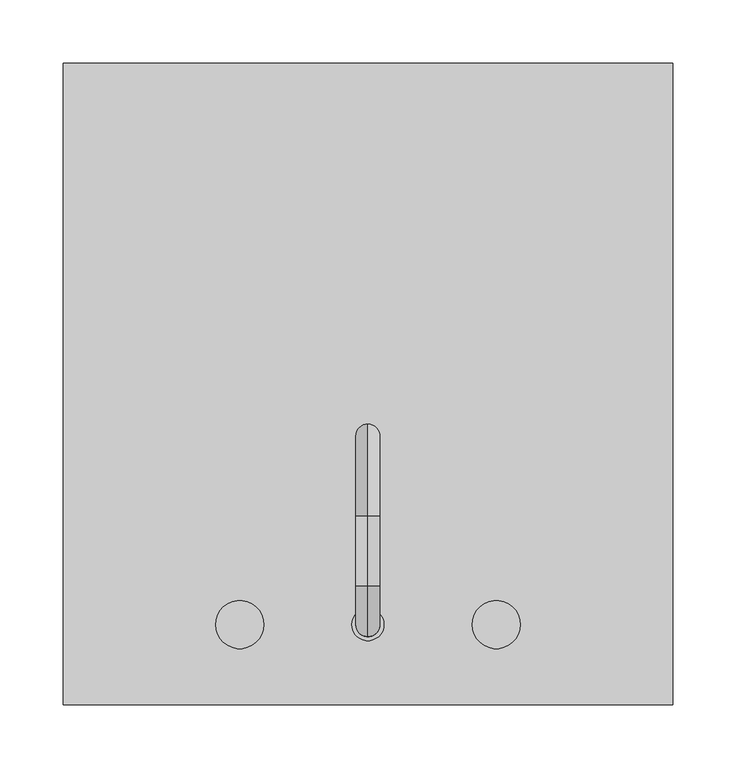
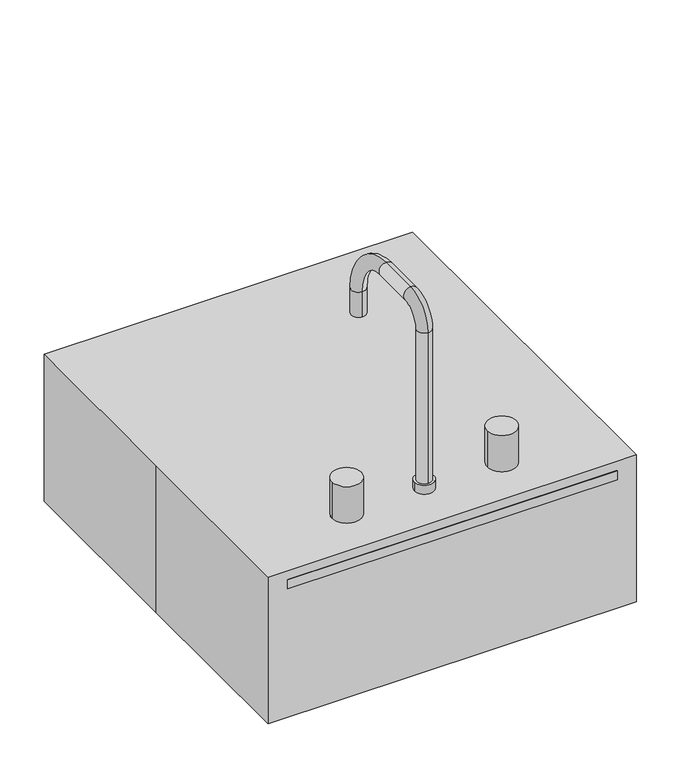
"""IFC4 building model written with IfcOpenShell, lengths in millimetres: proxy geometry, CS040 - Sink, SS, Single Compartment, 7.5x14x14 ID : CS040 - Sink, SS, Single Compartment, 7.5x14x14 ID."""

from ifc_helpers import new_model, si_unit, point, frame, frame_2d, origin, origin_with_axes, place, context, project, spatial, polyline, circle_curve, ellipse_curve, trimmed, segment, composite_curve, outline, extrude, source, transform, mapped, element, save
from ifc_brep_helpers import plane_surface, cylinder_surface, revolved_surface, advanced_brep


def specialty_equipment_c9b423af(model_context):
    return source(origin(), model_context, "Body", "SolidModel", [
        advanced_brep(
        [(-215.9, 215.9, 190.5), (-215.9, -254.0, 190.5), (215.9, -254.0, 190.5), (215.9, 215.9, 190.5), (133.35, -139.7, 190.5), (-133.35, -139.7, 190.5), (-177.8, -95.25, 190.5), (-177.8, 133.35, 190.5), (-133.35, 177.8, 190.5), (133.35, 177.8, 190.5), (177.8, 133.35, 190.5), (177.8, -95.25, 190.5), (-120.65, -190.5, 190.5), (-82.55, -190.5, 190.5), (-19.05, -190.5, 190.5), (19.05, -190.5, 190.5), (82.55, -190.5, 190.5), (120.65, -190.5, 190.5), (-215.9, 215.9, 177.8), (215.9, 215.9, 177.8), (215.9, -254.0, 177.8), (-215.9, -254.0, 177.8), (-120.65, -190.5, 177.8), (-82.55, -190.5, 177.8), (-19.05, -190.5, 177.8), (19.05, -190.5, 177.8), (82.55, -190.5, 177.8), (120.65, -190.5, 177.8), (184.15, -95.25, 177.8), (184.15, 133.35, 177.8), (133.35, 184.15, 177.8), (-133.35, 184.15, 177.8), (-184.15, 133.35, 177.8), (-184.15, -95.25, 177.8), (-133.35, -146.05, 177.8), (133.35, -146.05, 177.8), (177.8, -95.25, 177.8), (133.35, -139.7, 177.8), (177.8, 133.35, 177.8), (177.8, 133.35, 6.35), (177.8, -95.25, 6.35), (133.35, 177.8, 177.8), (-133.35, 177.8, 177.8), (-133.35, 177.8, 6.35), (133.35, 177.8, 6.35), (-177.8, 133.35, 177.8), (-177.8, -95.25, 177.8), (-177.8, -95.25, 6.35), (-177.8, 133.35, 6.35), (-133.35, -139.7, 177.8), (133.35, -139.7, 6.35), (-133.35, -139.7, 6.35), (184.15, -95.25, 0.0), (133.35, -146.05, 0.0), (184.15, 133.35, 0.0), (133.35, 184.15, 0.0), (-133.35, 184.15, 0.0), (-184.15, 133.35, 0.0), (-184.15, -95.25, 0.0), (-133.35, -146.05, 0.0), (-19.05, 19.05, 0.0), (19.05, 19.05, 0.0), (-19.05, 19.05, 6.35), (19.05, 19.05, 6.35)],
        [
            (0, 1),
            (1, 2),
            (2, 3),
            (3, 0),
            (4, 5),
            (5, 6, circle_curve(frame((-133.35, -95.25, 190.5), z_axis=(0.0, 0.0, -1.0), x_axis=(1.0, 0.0, 0.0)), 44.45)),
            (6, 7),
            (7, 8, circle_curve(frame((-133.35, 133.35, 190.5), z_axis=(0.0, 0.0, -1.0), x_axis=(1.0, 0.0, 0.0)), 44.45)),
            (8, 9),
            (9, 10, circle_curve(frame((133.35, 133.35, 190.5), z_axis=(0.0, 0.0, -1.0), x_axis=(1.0, 0.0, 0.0)), 44.45)),
            (10, 11),
            (11, 4, circle_curve(frame((133.35, -95.25, 190.5), z_axis=(0.0, 0.0, -1.0), x_axis=(1.0, 0.0, 0.0)), 44.45)),
            (12, 13, circle_curve(frame((-101.6, -190.5, 190.5), z_axis=(0.0, 0.0, -1.0), x_axis=(1.0, 0.0, 0.0)), 19.05)),
            (13, 12, circle_curve(frame((-101.6, -190.5, 190.5), z_axis=(0.0, 0.0, -1.0), x_axis=(1.0, 0.0, 0.0)), 19.05)),
            (14, 15, circle_curve(frame((0.0, -190.5, 190.5), z_axis=(0.0, 0.0, -1.0), x_axis=(1.0, 0.0, 0.0)), 19.05)),
            (15, 14, circle_curve(frame((0.0, -190.5, 190.5), z_axis=(0.0, 0.0, -1.0), x_axis=(1.0, 0.0, 0.0)), 19.05)),
            (16, 17, circle_curve(frame((101.6, -190.5, 190.5), z_axis=(0.0, 0.0, -1.0), x_axis=(1.0, 0.0, 0.0)), 19.05)),
            (17, 16, circle_curve(frame((101.6, -190.5, 190.5), z_axis=(0.0, 0.0, -1.0), x_axis=(1.0, 0.0, 0.0)), 19.05)),
            (18, 19),
            (19, 20),
            (20, 21),
            (21, 18),
            (22, 23, circle_curve(frame((-101.6, -190.5, 177.8), z_axis=(0.0, 0.0, 1.0), x_axis=(1.0, 0.0, 0.0)), 19.05)),
            (23, 22, circle_curve(frame((-101.6, -190.5, 177.8), z_axis=(0.0, 0.0, 1.0), x_axis=(1.0, 0.0, 0.0)), 19.05)),
            (24, 25, circle_curve(frame((0.0, -190.5, 177.8), z_axis=(0.0, 0.0, 1.0), x_axis=(1.0, 0.0, 0.0)), 19.05)),
            (25, 24, circle_curve(frame((0.0, -190.5, 177.8), z_axis=(0.0, 0.0, 1.0), x_axis=(1.0, 0.0, 0.0)), 19.05)),
            (26, 27, circle_curve(frame((101.6, -190.5, 177.8), z_axis=(0.0, 0.0, 1.0), x_axis=(1.0, 0.0, 0.0)), 19.05)),
            (27, 26, circle_curve(frame((101.6, -190.5, 177.8), z_axis=(0.0, 0.0, 1.0), x_axis=(1.0, 0.0, 0.0)), 19.05)),
            (28, 29),
            (29, 30, circle_curve(frame((133.35, 133.35, 177.8), z_axis=(0.0, 0.0, 1.0), x_axis=(1.0, 0.0, 0.0)), 50.8)),
            (30, 31),
            (31, 32, circle_curve(frame((-133.35, 133.35, 177.8), z_axis=(0.0, 0.0, 1.0), x_axis=(0.0, 1.0, 0.0)), 50.8)),
            (32, 33),
            (33, 34, circle_curve(frame((-133.35, -95.25, 177.8), z_axis=(0.0, 0.0, 1.0), x_axis=(-1.0, 0.0, 0.0)), 50.8)),
            (34, 35),
            (35, 28, circle_curve(frame((133.35, -95.25, 177.8), z_axis=(0.0, 0.0, 1.0), x_axis=(0.0, -1.0, 0.0)), 50.8)),
            (3, 19),
            (18, 0),
            (2, 20),
            (1, 21),
            (11, 36),
            (36, 37, circle_curve(frame((133.35, -95.25, 177.8), z_axis=(0.0, 0.0, -1.0), x_axis=(1.0, 0.0, 0.0)), 44.45)),
            (37, 4),
            (10, 38),
            (38, 39),
            (39, 40),
            (40, 36),
            (9, 41),
            (41, 38, circle_curve(frame((133.35, 133.35, 177.8), z_axis=(0.0, 0.0, -1.0), x_axis=(1.0, 0.0, 0.0)), 44.45)),
            (8, 42),
            (42, 43),
            (43, 44),
            (44, 41),
            (7, 45),
            (45, 42, circle_curve(frame((-133.35, 133.35, 177.8), z_axis=(0.0, 0.0, -1.0), x_axis=(1.0, 0.0, 0.0)), 44.45)),
            (6, 46),
            (46, 47),
            (47, 48),
            (48, 45),
            (5, 49),
            (49, 46, circle_curve(frame((-133.35, -95.25, 177.8), z_axis=(0.0, 0.0, -1.0), x_axis=(1.0, 0.0, 0.0)), 44.45)),
            (37, 50),
            (50, 51),
            (51, 49),
            (13, 23),
            (22, 12),
            (15, 25),
            (24, 14),
            (17, 27),
            (26, 16),
            (52, 28),
            (35, 53),
            (53, 52, circle_curve(frame((133.35, -95.25, 0.0), z_axis=(0.0, 0.0, 1.0), x_axis=(0.0, -1.0, 0.0)), 50.8)),
            (40, 50, circle_curve(frame((133.35, -95.25, 6.35), z_axis=(0.0, 0.0, -1.0), x_axis=(0.0, -1.0, 0.0)), 44.45)),
            (52, 54),
            (54, 29),
            (54, 55, circle_curve(frame((133.35, 133.35, 0.0), z_axis=(0.0, 0.0, 1.0), x_axis=(1.0, 0.0, 0.0)), 50.8)),
            (55, 30),
            (44, 39, circle_curve(frame((133.35, 133.35, 6.35), z_axis=(0.0, 0.0, -1.0), x_axis=(1.0, 0.0, 0.0)), 44.45)),
            (55, 56),
            (56, 31),
            (56, 57, circle_curve(frame((-133.35, 133.35, 0.0), z_axis=(0.0, 0.0, 1.0), x_axis=(0.0, 1.0, 0.0)), 50.8)),
            (57, 32),
            (48, 43, circle_curve(frame((-133.35, 133.35, 6.35), z_axis=(0.0, 0.0, -1.0), x_axis=(0.0, 1.0, 0.0)), 44.45)),
            (57, 58),
            (58, 33),
            (58, 59, circle_curve(frame((-133.35, -95.25, 0.0), z_axis=(0.0, 0.0, 1.0), x_axis=(-1.0, 0.0, 0.0)), 50.8)),
            (59, 34),
            (51, 47, circle_curve(frame((-133.35, -95.25, 6.35), z_axis=(0.0, 0.0, -1.0), x_axis=(-1.0, 0.0, 0.0)), 44.45)),
            (59, 53),
            (60, 61, circle_curve(frame((0.0, 19.05, 0.0), z_axis=(0.0, 0.0, 1.0), x_axis=(1.0, 0.0, 0.0)), 19.05)),
            (61, 60, circle_curve(frame((0.0, 19.05, 0.0), z_axis=(0.0, 0.0, 1.0), x_axis=(1.0, 0.0, 0.0)), 19.05)),
            (62, 63, circle_curve(frame((0.0, 19.05, 6.35), z_axis=(0.0, 0.0, -1.0), x_axis=(1.0, 0.0, 0.0)), 19.05)),
            (63, 62, circle_curve(frame((0.0, 19.05, 6.35), z_axis=(0.0, 0.0, -1.0), x_axis=(1.0, 0.0, 0.0)), 19.05)),
            (63, 61),
            (60, 62),
        ],
        [
            plane_surface(frame((215.9, 215.9, 190.5), z_axis=(0.0, 0.0, 1.0), x_axis=(1.0, 0.0, 0.0))),
            plane_surface(frame((215.9, 215.9, 177.8), z_axis=(0.0, 0.0, -1.0), x_axis=(-1.0, 0.0, 0.0))),
            plane_surface(frame((-215.9, 215.9, 190.5), z_axis=(0.0, 1.0, 0.0), x_axis=(0.0, 0.0, -1.0))),
            plane_surface(frame((215.9, 215.9, 190.5), z_axis=(1.0, 0.0, 0.0), x_axis=(0.0, 0.0, -1.0))),
            plane_surface(frame((215.9, -254.0, 190.5), z_axis=(0.0, -1.0, 0.0), x_axis=(0.0, 0.0, -1.0))),
            plane_surface(frame((-215.9, -254.0, 190.5), z_axis=(-1.0, 0.0, 0.0), x_axis=(0.0, 0.0, -1.0))),
            revolved_surface(polyline([(177.8, -95.25, 177.8), (177.8, -95.25, 190.5)]), (133.35, -95.25, 177.8), (0.0, 0.0, -1.0)),
            plane_surface(frame((177.8, -95.25, 190.5), z_axis=(-1.0, 0.0, 0.0), x_axis=(0.0, 0.0, -1.0))),
            revolved_surface(polyline([(177.8, 133.35, 177.8), (177.8, 133.35, 190.5)]), (133.35, 133.35, 177.8), (0.0, 0.0, -1.0)),
            plane_surface(frame((133.35, 177.8, 190.5), z_axis=(0.0, -1.0, 0.0), x_axis=(0.0, 0.0, -1.0))),
            revolved_surface(polyline([(-88.89999999999999, 133.35, 177.8), (-88.89999999999999, 133.35, 190.5)]), (-133.35, 133.35, 177.8), (0.0, 0.0, -1.0)),
            plane_surface(frame((-177.8, 133.35, 190.5), z_axis=(1.0, 0.0, 0.0), x_axis=(0.0, 0.0, -1.0))),
            revolved_surface(polyline([(-88.89999999999999, -95.25, 177.8), (-88.89999999999999, -95.25, 190.5)]), (-133.35, -95.25, 177.8), (0.0, 0.0, -1.0)),
            plane_surface(frame((-133.35, -139.7, 190.5), z_axis=(0.0, 1.0, 0.0), x_axis=(0.0, 0.0, -1.0))),
            revolved_surface(polyline([(-82.55, -190.5, 177.8), (-82.55, -190.5, 190.5)]), (-101.6, -190.5, 177.8), (0.0, 0.0, -1.0)),
            revolved_surface(polyline([(19.05, -190.5, 177.8), (19.05, -190.5, 190.5)]), (0.0, -190.5, 177.8), (0.0, 0.0, -1.0)),
            revolved_surface(polyline([(120.64999999999999, -190.5, 177.8), (120.64999999999999, -190.5, 190.5)]), (101.6, -190.5, 177.8), (0.0, 0.0, -1.0)),
            cylinder_surface(frame((133.35, -95.25, 190.5), z_axis=(0.0, 0.0, -1.0), x_axis=(0.0, -1.0, 0.0)), 50.8),
            revolved_surface(polyline([(133.35, -139.7, 6.349999999999994), (133.35, -139.7, 177.8)]), (133.35, -95.25, 190.5), (0.0, 0.0, -1.0)),
            plane_surface(frame((184.15, -95.25, 177.8), z_axis=(1.0, 0.0, 0.0), x_axis=(0.0, 1.0, 0.0))),
            cylinder_surface(frame((133.35, 133.35, 190.5), z_axis=(0.0, 0.0, -1.0), x_axis=(1.0, 0.0, 0.0)), 50.8),
            revolved_surface(polyline([(177.8, 133.35, 6.349999999999994), (177.8, 133.35, 177.8)]), (133.35, 133.35, 190.5), (0.0, 0.0, -1.0)),
            plane_surface(frame((133.35, 184.15, 177.8), z_axis=(0.0, 1.0, 0.0), x_axis=(-1.0, 0.0, 0.0))),
            cylinder_surface(frame((-133.35, 133.35, 190.5), z_axis=(0.0, 0.0, -1.0), x_axis=(0.0, 1.0, 0.0)), 50.8),
            revolved_surface(polyline([(-133.35, 177.8, 6.349999999999994), (-133.35, 177.8, 177.8)]), (-133.35, 133.35, 190.5), (0.0, 0.0, -1.0)),
            plane_surface(frame((-184.15, 133.35, 177.8), z_axis=(-1.0, 0.0, 0.0), x_axis=(0.0, -1.0, 0.0))),
            cylinder_surface(frame((-133.35, -95.25, 190.5), z_axis=(0.0, 0.0, -1.0), x_axis=(-1.0, 0.0, 0.0)), 50.8),
            revolved_surface(polyline([(-177.8, -95.25, 6.349999999999994), (-177.8, -95.25, 177.8)]), (-133.35, -95.25, 190.5), (0.0, 0.0, -1.0)),
            plane_surface(frame((-133.35, -146.05, 177.8), z_axis=(0.0, -1.0, 0.0), x_axis=(1.0, 0.0, 0.0))),
            plane_surface(frame((-133.35, -146.05, 0.0), z_axis=(0.0, 0.0, -1.0), x_axis=(1.0, 0.0, 0.0))),
            plane_surface(frame((-88.9, -95.25, 6.35), z_axis=(0.0, 0.0, 1.0), x_axis=(0.0, -1.0, 0.0))),
            revolved_surface(polyline([(19.05, 19.05, 0.0), (19.05, 19.05, 6.35)]), (0.0, 19.05, 0.0), (0.0, 0.0, -1.0)),
        ],
        [
            (0, [[1, 2, 3, 4], [5, 6, 7, 8, 9, 10, 11, 12], [13, 14], [15, 16], [17, 18]]),
            (1, [[19, 20, 21, 22], [23, 24], [25, 26], [27, 28], [29, 30, 31, 32, 33, 34, 35, 36]]),
            (2, [[37, -19, 38, -4]]),
            (3, [[39, -20, -37, -3]]),
            (4, [[40, -21, -39, -2]]),
            (5, [[-38, -22, -40, -1]]),
            (6, [[41, 42, 43, -12]]),
            (7, [[44, 45, 46, 47, -41, -11]]),
            (8, [[48, 49, -44, -10]]),
            (9, [[50, 51, 52, 53, -48, -9]]),
            (10, [[54, 55, -50, -8]]),
            (11, [[56, 57, 58, 59, -54, -7]]),
            (12, [[60, 61, -56, -6]]),
            (13, [[-43, 62, 63, 64, -60, -5]]),
            (14, [[65, -23, 66, -14]]),
            (14, [[-66, -24, -65, -13]]),
            (15, [[67, -25, 68, -16]]),
            (15, [[-68, -26, -67, -15]]),
            (16, [[69, -27, 70, -18]]),
            (16, [[-70, -28, -69, -17]]),
            (17, [[71, -36, 72, 73]]),
            (18, [[-47, 74, -62, -42]]),
            (19, [[75, 76, -29, -71]]),
            (20, [[77, 78, -30, -76]]),
            (21, [[-53, 79, -45, -49]]),
            (22, [[80, 81, -31, -78]]),
            (23, [[82, 83, -32, -81]]),
            (24, [[-59, 84, -51, -55]]),
            (25, [[85, 86, -33, -83]]),
            (26, [[87, 88, -34, -86]]),
            (27, [[-64, 89, -57, -61]]),
            (28, [[-35, -88, 90, -72]]),
            (29, [[-90, -87, -85, -82, -80, -77, -75, -73], [91, 92]]),
            (30, [[-79, -52, -84, -58, -89, -63, -74, -46], [93, 94]]),
            (31, [[95, -91, 96, -94]]),
            (31, [[-96, -92, -95, -93]]),
        ],
    ),
        extrude(outline(polyline([(-241.3, -254.0), (-241.3, 0.0), (-241.3, 254.0), (241.3, 254.0), (241.3, -254.0), (-241.3, -254.0)])), origin_with_axes(), (0.0, 0.0, 1.0), 203.2),
        advanced_brep(
        [(0.0, -200.025, 203.2), (0.0, -180.975, 203.2), (0.0, -180.975, 423.8625), (0.0, -200.025, 423.8625), (0.0, -160.3375, 444.5), (0.0, -160.3375, 463.55), (0.0, -104.775, 444.5), (0.0, -104.775, 463.55), (0.0, -50.8, 390.525), (0.0, -31.75, 390.525), (0.0, -31.75, 355.6), (0.0, -50.8, 355.6)],
        [
            (0, 1, circle_curve(frame((0.0, -190.5, 203.2), z_axis=(0.0, 0.0, -1.0), x_axis=(0.0, 1.0, 0.0)), 9.525)),
            (1, 0, circle_curve(frame((0.0, -190.5, 203.2), z_axis=(0.0, 0.0, -1.0), x_axis=(0.0, 1.0, 0.0)), 9.525)),
            (1, 2),
            (2, 3, circle_curve(frame((0.0, -190.5, 423.8625), z_axis=(0.0, 0.0, -1.0), x_axis=(0.0, 1.0, 0.0)), 9.525)),
            (3, 0),
            (3, 2, circle_curve(frame((0.0, -190.5, 423.8625), z_axis=(0.0, 0.0, -1.0), x_axis=(0.0, 1.0, 0.0)), 9.525)),
            (4, 5, circle_curve(frame((0.0, -160.3375, 454.025), z_axis=(0.0, -1.0, 0.0), x_axis=(0.0, 0.0, -1.0)), 9.525)),
            (5, 3, circle_curve(frame((0.0, -160.3375, 423.8625), z_axis=(1.0, 0.0, 0.0), x_axis=(0.0, -1.0, 0.0)), 39.6875)),
            (2, 4, circle_curve(frame((0.0, -160.3375, 423.8625), z_axis=(-1.0, 0.0, 0.0), x_axis=(0.0, -1.0, 0.0)), 20.6375)),
            (5, 4, circle_curve(frame((0.0, -160.3375, 454.025), z_axis=(0.0, -1.0, 0.0), x_axis=(0.0, 0.0, -1.0)), 9.525)),
            (4, 6),
            (6, 7, circle_curve(frame((0.0, -104.775, 454.025), z_axis=(0.0, -1.0, 0.0), x_axis=(0.0, 0.0, -1.0)), 9.525)),
            (7, 5),
            (7, 6, circle_curve(frame((0.0, -104.775, 454.025), z_axis=(0.0, -1.0, 0.0), x_axis=(0.0, 0.0, -1.0)), 9.525)),
            (8, 9, circle_curve(frame((0.0, -41.275, 390.525), z_axis=(0.0, 0.0, 1.0), x_axis=(0.0, -1.0, 0.0)), 9.525)),
            (9, 7, circle_curve(frame((0.0, -104.775, 390.525), z_axis=(1.0, 0.0, 0.0), x_axis=(0.0, 0.0, 1.0)), 73.025)),
            (6, 8, circle_curve(frame((0.0, -104.775, 390.525), z_axis=(-1.0, 0.0, 0.0), x_axis=(0.0, 0.0, 1.0)), 53.975)),
            (9, 8, circle_curve(frame((0.0, -41.275, 390.525), z_axis=(0.0, 0.0, 1.0), x_axis=(0.0, -1.0, 0.0)), 9.525)),
            (10, 11, circle_curve(frame((0.0, -41.275, 355.6), z_axis=(0.0, 0.0, -1.0), x_axis=(0.0, -1.0, 0.0)), 9.525)),
            (11, 10, circle_curve(frame((0.0, -41.275, 355.6), z_axis=(0.0, 0.0, -1.0), x_axis=(0.0, -1.0, 0.0)), 9.525)),
            (8, 11),
            (10, 9),
        ],
        [
            plane_surface(frame((0.0, -180.975, 203.2), z_axis=(0.0, 0.0, -1.0), x_axis=(1.0, 0.0, 0.0))),
            cylinder_surface(frame((0.0, -190.5, 203.2), z_axis=(0.0, 0.0, -1.0), x_axis=(0.0, 1.0, 0.0)), 9.525),
            revolved_surface(trimmed(ellipse_curve(frame((0.0, -190.5, 423.8625), z_axis=(0.0, 0.0, 1.0), x_axis=(0.0, 1.0, 0.0)), 9.525, 9.525), [point((0.0, -200.025, 423.8625))], [point((0.0, -180.975, 423.8625))], True, "CARTESIAN"), (0.0, -160.3375, 423.8625), (1.0, 0.0, 0.0)),
            revolved_surface(trimmed(ellipse_curve(frame((0.0, -190.5, 423.8625), z_axis=(0.0, 0.0, 1.0), x_axis=(0.0, 1.0, 0.0)), 9.525, 9.525), [point((0.0, -180.975, 423.8625))], [point((0.0, -200.025, 423.8625))], True, "CARTESIAN"), (0.0, -160.3375, 423.8625), (1.0, 0.0, 0.0)),
            cylinder_surface(frame((0.0, -160.3375, 454.025), z_axis=(0.0, -1.0, 0.0), x_axis=(0.0, 0.0, -1.0)), 9.525),
            revolved_surface(trimmed(ellipse_curve(frame((0.0, -104.775, 454.025), z_axis=(0.0, 1.0, 0.0), x_axis=(0.0, 0.0, -1.0)), 9.525, 9.525), [point((0.0, -104.775, 463.55))], [point((0.0, -104.775, 444.5))], True, "CARTESIAN"), (0.0, -104.775, 390.525), (1.0, 0.0, 0.0)),
            revolved_surface(trimmed(ellipse_curve(frame((0.0, -104.775, 454.025), z_axis=(0.0, 1.0, 0.0), x_axis=(0.0, 0.0, -1.0)), 9.525, 9.525), [point((0.0, -104.775, 444.5))], [point((0.0, -104.775, 463.55))], True, "CARTESIAN"), (0.0, -104.775, 390.525), (1.0, 0.0, 0.0)),
            plane_surface(frame((0.0, -31.75, 355.6), z_axis=(0.0, 0.0, -1.0), x_axis=(-1.0, 0.0, 0.0))),
            cylinder_surface(frame((0.0, -41.275, 390.525), z_axis=(0.0, 0.0, 1.0), x_axis=(0.0, -1.0, 0.0)), 9.525),
        ],
        [
            (0, [[1, 2]]),
            (1, [[3, 4, 5, -2]]),
            (1, [[-5, 6, -3, -1]]),
            (2, [[7, 8, -4, 9]]),
            (3, [[10, -9, -6, -8]]),
            (4, [[11, 12, 13, -7]]),
            (4, [[-13, 14, -11, -10]]),
            (5, [[15, 16, -12, 17]]),
            (6, [[18, -17, -14, -16]]),
            (7, [[19, 20]]),
            (8, [[21, -19, 22, -15]]),
            (8, [[-22, -20, -21, -18]]),
        ],
    ),
        extrude(outline(composite_curve([segment(trimmed(circle_curve(frame_2d((0.0, -190.5)), 12.7), [point((-12.7, -190.5))], [point((12.7, -190.5))], False, "CARTESIAN"), True, "CONTINUOUS"), segment(trimmed(circle_curve(frame_2d((0.0, -190.5)), 12.7), [point((12.7, -190.5))], [point((-12.7, -190.5))], False, "CARTESIAN"), True, "CONTINUOUS")], self_intersect=False), holes=[composite_curve([segment(trimmed(circle_curve(frame_2d((0.0, -190.5)), 9.525), [point((-9.525, -190.5))], [point((9.525, -190.5))], True, "CARTESIAN"), True, "CONTINUOUS"), segment(trimmed(circle_curve(frame_2d((0.0, -190.5)), 9.525), [point((9.525, -190.5))], [point((-9.525, -190.5))], True, "CARTESIAN"), True, "CONTINUOUS")], self_intersect=False)]), frame((0.0, 0.0, 203.2), z_axis=(0.0, 0.0, 1.0), x_axis=(1.0, 0.0, 0.0)), (0.0, 0.0, 1.0), 12.7),
        extrude(outline(composite_curve([segment(trimmed(circle_curve(frame_2d((-101.6, -190.5)), 19.05), [point((-120.65, -190.5))], [point((-82.55, -190.5))], False, "CARTESIAN"), True, "CONTINUOUS"), segment(trimmed(circle_curve(frame_2d((-101.6, -190.5)), 19.05), [point((-82.55, -190.5))], [point((-120.65, -190.5))], False, "CARTESIAN"), True, "CONTINUOUS")], self_intersect=False)), frame((0.0, 0.0, 203.2), z_axis=(0.0, 0.0, 1.0), x_axis=(1.0, 0.0, 0.0)), (0.0, 0.0, 1.0), 50.8),
        extrude(outline(composite_curve([segment(trimmed(circle_curve(frame_2d((101.6, -190.5)), 19.05), [point((82.55, -190.5))], [point((120.65, -190.5))], False, "CARTESIAN"), True, "CONTINUOUS"), segment(trimmed(circle_curve(frame_2d((101.6, -190.5)), 19.05), [point((120.65, -190.5))], [point((82.55, -190.5))], False, "CARTESIAN"), True, "CONTINUOUS")], self_intersect=False)), frame((0.0, 0.0, 203.2), z_axis=(0.0, 0.0, 1.0), x_axis=(1.0, 0.0, 0.0)), (0.0, 0.0, 1.0), 50.8),
        extrude(outline(composite_curve([segment(polyline([(101.6, -209.55), (-101.6, -209.55)]), True, "CONTINUOUS"), segment(trimmed(circle_curve(frame_2d((-101.6, -190.5)), 19.05), [point((-101.6, -209.55))], [point((-101.6, -171.45))], False, "CARTESIAN"), True, "CONTINUOUS"), segment(polyline([(-101.6, -171.45), (101.6, -171.45)]), True, "CONTINUOUS"), segment(trimmed(circle_curve(frame_2d((101.6, -190.5)), 19.05), [point((101.6, -171.45))], [point((101.6, -209.55))], False, "CARTESIAN"), True, "CONTINUOUS")], self_intersect=False), holes=[composite_curve([segment(trimmed(circle_curve(frame_2d((0.0, -190.5)), 9.525), [point((-9.525, -190.5))], [point((9.525, -190.5))], True, "CARTESIAN"), True, "CONTINUOUS"), segment(trimmed(circle_curve(frame_2d((0.0, -190.5)), 9.525), [point((9.525, -190.5))], [point((-9.525, -190.5))], True, "CARTESIAN"), True, "CONTINUOUS")], self_intersect=False)]), frame((0.0, 0.0, 190.5), z_axis=(0.0, 0.0, 1.0), x_axis=(1.0, 0.0, 0.0)), (0.0, 0.0, 1.0), 12.7),
    ])


if __name__ == "__main__":
    model = new_model("IFC4")
    model_context = context("Model", 3, world=origin())
    ifc_project = project(units=[si_unit("LENGTHUNIT", "METRE", prefix="MILLI")], contexts=[model_context])
    site = spatial("IfcSite", under=ifc_project)
    building = spatial("IfcBuilding", under=site)
    placement = place(None, origin())
    specialty_equipment_shape = specialty_equipment_c9b423af(model_context)
    element("IfcBuildingElementProxy", 1, Name="CS040 - Sink, SS, Single Compartment, 7.5x14x14 ID : CS040 - Sink, SS, Single Compartment, 7.5x14x14 ID", ObjectType="CS040 - Sink, SS, Single Compartment, 7.5x14x14 ID : CS040 - Sink, SS, Single Compartment, 7.5x14x14 ID", at=placement, inside=building, context=model_context, shape_type="MappedRepresentation", body=[
        mapped(specialty_equipment_shape, transform((0.0, 0.0, 0.0), x_axis=(1.0, 0.0, 0.0), y_axis=(0.0, 1.0, 0.0), z_axis=(0.0, 0.0, 1.0))),
    ])
    save(model, "model.ifc")

# Revit data of these elements
# Type "CS040 - Sink, SS, Single Compartment, 7.5x14x14 ID : CS040 - Sink, SS, Single Compartment, 7.5x14x14 ID"
#   Watts2 = "0"
#   Watts1 = "0"
#   Unit_Issue = "EA"
#   UTIL_6_Misc = "-"
#   UTIL_5_NonMedGas = "-"
#   UTIL_4_MiscGas = "-"
#   UTIL_3_MedGas = "-"
#   UTIL_2_Elec = "-"
#   UTIL_1_WaterDrain = "D"
#   Nomenclature = "Sink, SS, Single Compartment, 7.5x14x14 ID"
#   NSN = "6530"
#   Location [instance default] = ""
#   JSN = "CS040"
#   Fund_Source_VA = "-"
#   Fund_Source_Navy = "-"
#   Fund_Source_Army = "-"
#   Fund_Source_AF = "-"
#   ELEC_Volts2 = "0"
#   ELEC_Volts1 = "0"
#   ELEC_Phase2 = "0"
#   ELEC_Phase1 = "0"
#   ELEC_HertzSwitch = "0"
#   ELEC_HertzDependent = "0"
#   ELEC_Hertz = "0"
#   ELEC_Amps2 = "0"
#   ELEC_Amps1 = "0"
#   DetailDescription = "Single compartment stainless steel sink, drop-in, self-rimming, ledge-type, connected with a drain and provided with a mixing faucet. It shall also be provided with pre-punched fixture holes on 4\" center, integral back ledge to accommodate deck-mounted fixtures, brushed/polished interior and top surfaces, and sound deadened. Recommended for use in suspended or U/C/B sink cabinets having a high plastic laminate or Chemsurf laminate countertop/work surface. Coordinate actual outside sink dimensions with the actual clear dimension of cabinet specified to ensure that they are compatible. For general purpose use throughout the facility."
#   CAT_VA = "A"
#   CAT_Navy = "A"
#   CAT_IHS = "-"
#   CAT_Army = "A"
#   CAT_AF = "A"
#   BTUperhour = "0"
#   Weight_IP = 19
#   DIM_Width_IP = 1' - 7"
#   DIM_Height_IP = 0' - 8"
#   DIM_Depth_IP = 1' - 8"
#   Faucet Material = Metal - Steel, Polished
# Element 1 (IfcBuildingElementProxy, "CS040 - Sink, SS, Single Compartment, 7.5x14x14 ID : CS040 - Sink, SS, Single Compartment, 7.5x14x14 ID")
#   Materials on its faces: "Metal - Steel, Polished", "EquipSpace"
# Materials
#   "Metal - Steel, Polished": class "Unassigned", colour RGB 57 57 57, transparency 0
#   "EquipSpace": class "Unassigned", colour RGB 221 217 195, transparency 0.5
